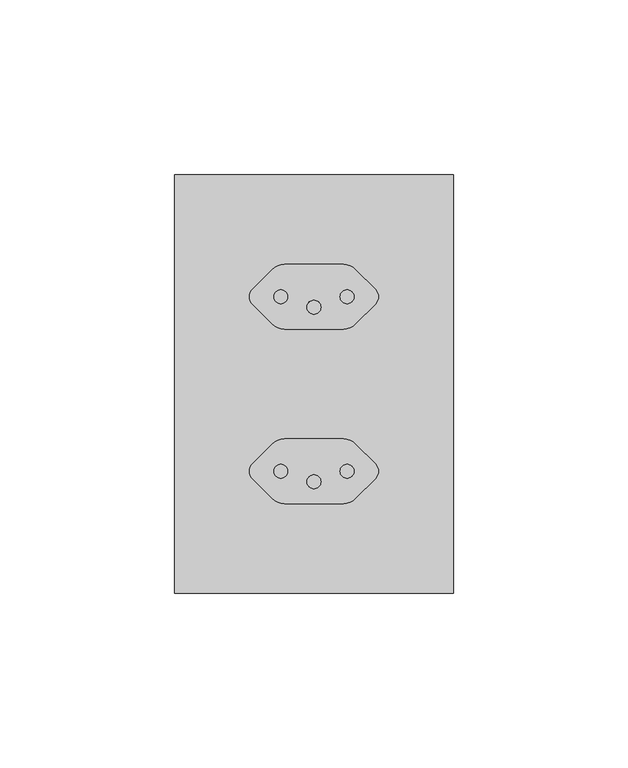
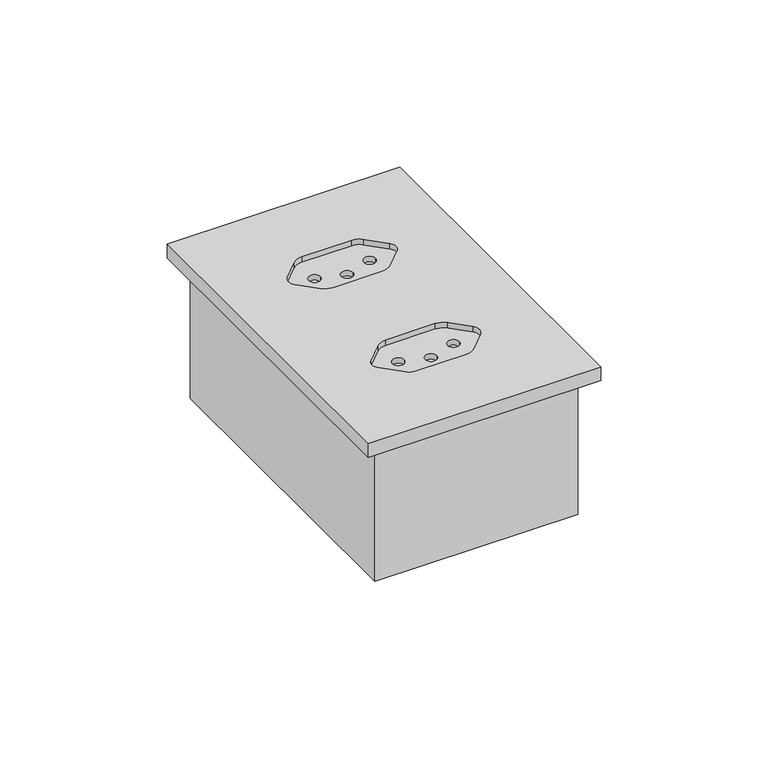
"""IFC4 building model written with IfcOpenShell, lengths in millimetres: proxy geometry, CAIXA VERTICE V7 : Tomada 10A 2s."""

import ifcopenshell
import ifcopenshell.guid

model = None  # the IFC model being written
_history = None  # IfcOwnerHistory: only IFC2X3 demands one
_inside = {}  # id of a spatial element -> (the spatial element, [elements in it])
_under = {}  # id of a project, library or spatial element -> (it, [spatial elements below it])
_declared = {}  # id of a project -> (the project, [libraries it declares])
_typed = {}  # id of a type object -> (the type object, [elements of that type])
_made_of = {}  # id of a material, layer set ... -> (it, [elements and type objects made of it])


def new_model(schema):
    """Start an empty IFC model of exactly this schema.

    Asked for "IFC4X3", IfcOpenShell would pick the latest addendum, in which some entities
    have other attributes; the version numbers below select the first issue.
    IFC2X3 requires an IfcOwnerHistory on every rooted entity: one is made here for all.
    """
    global model, _history
    if schema == "IFC4X3":
        model = ifcopenshell.file(schema_version=(4, 3, 0, 0))
    else:
        model = ifcopenshell.file(schema=schema)
    _inside.clear()
    _under.clear()
    _declared.clear()
    _typed.clear()
    _made_of.clear()
    _history = None
    if model.schema == "IFC2X3":
        org = make("IfcOrganization", Name="unknown")
        user = make(
            "IfcPersonAndOrganization",
            ThePerson=make("IfcPerson", FamilyName="unknown"),
            TheOrganization=org,
        )
        app = make(
            "IfcApplication",
            ApplicationDeveloper=org,
            Version="unknown",
            ApplicationFullName="unknown",
            ApplicationIdentifier="unknown",
        )
        _history = make(
            "IfcOwnerHistory",
            OwningUser=user,
            OwningApplication=app,
            ChangeAction="ADDED",
            CreationDate=0,
        )
    return model


def make(cls, **values):
    """One entity of the class cls with the attributes given. An attribute that is None is left unset."""
    return model.create_entity(
        cls, **{name: value for name, value in values.items() if value is not None}
    )


def rooted(cls, **values):
    """An entity with a GlobalId (a new one), such as an element, a storey or a relation."""
    return make(cls, GlobalId=ifcopenshell.guid.new(), OwnerHistory=_history, **values)


def si_unit(unit_type, name, prefix=None):
    """IfcSIUnit, for example si_unit("LENGTHUNIT", "METRE", prefix="MILLI")."""
    return make("IfcSIUnit", UnitType=unit_type, Prefix=prefix, Name=name)


def assignment(units):
    """IfcUnitAssignment: the units of a project."""
    return None if units is None else make("IfcUnitAssignment", Units=units)


def point(xyz):
    """IfcCartesianPoint."""
    return None if xyz is None else make("IfcCartesianPoint", Coordinates=xyz)


def direction(xyz):
    """IfcDirection."""
    return None if xyz is None else make("IfcDirection", DirectionRatios=xyz)


def frame(location, z_axis=None, x_axis=None):
    """IfcAxis2Placement3D, a coordinate frame: its origin and axes. An axis left out is left unset."""
    return make(
        "IfcAxis2Placement3D",
        Location=point(location),
        Axis=direction(z_axis),
        RefDirection=direction(x_axis),
    )


def origin():
    """The frame at (0, 0, 0) with its axes left unset."""
    return frame((0.0, 0.0, 0.0))


def place(relative_to, where):
    """IfcLocalPlacement: puts the frame where relative to a parent placement (None: the world)."""
    return make(
        "IfcLocalPlacement", PlacementRelTo=relative_to, RelativePlacement=where
    )


def context(
    kind, dimensions, precision=None, world=None, true_north=None, identifier=None
):
    """IfcGeometricRepresentationContext, for example the 3D "Model" context."""
    return make(
        "IfcGeometricRepresentationContext",
        ContextIdentifier=identifier,
        ContextType=kind,
        CoordinateSpaceDimension=dimensions,
        Precision=precision,
        WorldCoordinateSystem=world,
        TrueNorth=true_north,
    )


def project(units=None, contexts=None):
    """IfcProject with its units and contexts."""
    return rooted(
        "IfcProject",
        Name="project",
        RepresentationContexts=contexts,
        UnitsInContext=assignment(units),
    )


def spatial(cls, under=None, at=None, **own):
    """A site, building, storey or space (cls), placed at a placement, below another one or the project."""
    s = rooted(cls, ObjectPlacement=at, **own)
    if under is not None:
        _under.setdefault(under.id(), (under, []))[1].append(s)
    return s


def polyline(points):
    """IfcPolyline through the points."""
    return make("IfcPolyline", Points=[point(p) for p in points])


def circle_curve(where, radius):
    """IfcCircle in the frame where."""
    return make("IfcCircle", Position=where, Radius=radius)


def faces_of(points, faces, orient=None, outer=None):
    """IfcFace entities. A face is a list of loops; a loop is a list of indices into points, from 0.

    orient and outer hold one flag for each loop. By default every Orientation is true, the
    first loop of a face is its IfcFaceOuterBound and the others are IfcFaceBound.
    """
    made = []
    for i, loops in enumerate(faces):
        bounds = []
        for j, loop in enumerate(loops):
            is_outer = j == 0 if outer is None else outer[i][j]
            bounds.append(
                make(
                    "IfcFaceOuterBound" if is_outer else "IfcFaceBound",
                    Bound=make("IfcPolyLoop", Polygon=[points[k] for k in loop]),
                    Orientation=True if orient is None else orient[i][j],
                )
            )
        made.append(make("IfcFace", Bounds=bounds))
    return made


def faceted_brep(points, faces, orient=None, outer=None, voids=None):
    """IfcFacetedBrep: a solid bounded by flat faces; with voids (closed shells), ...WithVoids."""
    shared = [point(p) for p in points]
    hull = make("IfcClosedShell", CfsFaces=faces_of(shared, faces, orient, outer))
    if voids is None:
        return make("IfcFacetedBrep", Outer=hull)
    return make(
        "IfcFacetedBrepWithVoids",
        Outer=hull,
        Voids=[
            make(cls, CfsFaces=faces_of(shared, fs, o, b)) for cls, fs, o, b in voids
        ],
    )


def shape(context_of_items, identifier, shape_type, items):
    """IfcShapeRepresentation: the items that make up one representation, for example the "Body"."""
    return make(
        "IfcShapeRepresentation",
        ContextOfItems=context_of_items,
        RepresentationIdentifier=identifier,
        RepresentationType=shape_type,
        Items=items,
    )


def source(mapping_origin, context_of_items, identifier, shape_type, items):
    """IfcRepresentationMap: a shape defined once, which mapped items show again and again."""
    return make(
        "IfcRepresentationMap",
        MappingOrigin=mapping_origin,
        MappedRepresentation=shape(context_of_items, identifier, shape_type, items),
    )


def transform(
    local_origin,
    x_axis=None,
    y_axis=None,
    z_axis=None,
    scale=None,
    scale2=None,
    scale3=None,
    uniform=True,
):
    """IfcCartesianTransformationOperator3D, or its non-uniform kind. x_axis, y_axis, z_axis: its Axis1, 2, 3."""
    if uniform:
        return make(
            "IfcCartesianTransformationOperator3D",
            Axis1=direction(x_axis),
            Axis2=direction(y_axis),
            LocalOrigin=point(local_origin),
            Scale=scale,
            Axis3=direction(z_axis),
        )
    return make(
        "IfcCartesianTransformationOperator3DnonUniform",
        Axis1=direction(x_axis),
        Axis2=direction(y_axis),
        LocalOrigin=point(local_origin),
        Scale=scale,
        Axis3=direction(z_axis),
        Scale2=scale2,
        Scale3=scale3,
    )


def mapped(mapping_source, mapping_target):
    """IfcMappedItem: shows the shape of a source again, moved by a transform."""
    return make(
        "IfcMappedItem", MappingSource=mapping_source, MappingTarget=mapping_target
    )


def made_of(thing, what):
    """Note that an element or type object is made of a material, layer set ...; save() writes the relation."""
    if what is not None:
        _made_of.setdefault(what.id(), (what, []))[1].append(thing)
    return thing


def element(
    cls,
    number,
    at=None,
    inside=None,
    cuts=None,
    type_object=None,
    material=None,
    context=None,
    identifier="Body",
    shape_type=None,
    held_by="IfcProductDefinitionShape",
    body=None,
    shapes=None,
    **own,
):
    """One element of the class cls, such as IfcWall. Its Tag is "e" and its number.

    at: its placement. inside: the storey or other place that contains it. cuts: it is an
    opening in that element (IfcRelVoidsElement). A single representation is given by context,
    identifier, shape_type and body (its items); several are given by shapes. held_by: the class
    of the entity that holds the representations. save() writes the other relations.
    """
    e = rooted(cls, Tag="e%d" % number, ObjectPlacement=at, **own)
    if body is not None:
        shapes = [shape(context, identifier, shape_type, body)]
    if shapes is not None:
        e.Representation = make(held_by, Representations=shapes)
    if inside is not None:
        _inside.setdefault(inside.id(), (inside, []))[1].append(e)
    if cuts is not None:
        rooted(
            "IfcRelVoidsElement", RelatingBuildingElement=cuts, RelatedOpeningElement=e
        )
    if type_object is not None:
        _typed.setdefault(type_object.id(), (type_object, []))[1].append(e)
    return made_of(e, material)


def aggregate(whole, parts):
    """IfcRelAggregates: a whole, such as a stair, and the parts it consists of."""
    return rooted("IfcRelAggregates", RelatingObject=whole, RelatedObjects=parts)


def save(model, path):
    """Write the relations noted so far, then the file.

    IfcRelAggregates (storeys below a building ...), IfcRelContainedInSpatialStructure (elements
    in a storey), IfcRelDefinesByType, IfcRelAssociatesMaterial and IfcRelDeclares: one each for
    every whole, place, type object, material and project.
    """
    for whole, parts in _under.values():
        aggregate(whole, parts)
    for where, things in _inside.values():
        rooted(
            "IfcRelContainedInSpatialStructure",
            RelatedElements=things,
            RelatingStructure=where,
        )
    for kind, things in _typed.values():
        rooted("IfcRelDefinesByType", RelatedObjects=things, RelatingType=kind)
    for what, things in _made_of.values():
        rooted("IfcRelAssociatesMaterial", RelatedObjects=things, RelatingMaterial=what)
    for by, libraries in _declared.values():
        rooted("IfcRelDeclares", RelatingContext=by, RelatedDefinitions=libraries)
    model.write(path)


def plane_surface(at):
    """IfcPlane: the flat surface through the origin of the frame at, square to its z axis."""
    return make("IfcPlane", Position=at)


def revolved_surface(curve, axis_point, axis_direction):
    """IfcSurfaceOfRevolution: the curve turned about the line through axis_point along axis_direction."""
    return make(
        "IfcSurfaceOfRevolution",
        SweptCurve=make("IfcArbitraryOpenProfileDef", ProfileType="CURVE", Curve=curve),
        AxisPosition=make("IfcAxis1Placement", Location=point(axis_point), Axis=direction(axis_direction)),
    )


def advanced_brep(points, edges, surfaces, faces):
    """IfcAdvancedBrep: a solid bounded by faces that lie on surfaces and meet in shared edges.

    An edge is (start, end): straight between two places in points (the first is 0);
    or (start, end, curve); or (start, end, curve, False) where it runs against its curve.
    A face is (place in surfaces, loops), or (place, loops, False) where it looks against
    its surface's normal. A loop lists edges by number (the first is 1), with a minus sign
    where the edge is run from its end to its start. The first loop is the outer one.
    """
    corners = [point(p) for p in points]
    vertices = [make("IfcVertexPoint", VertexGeometry=c) for c in corners]
    made = []
    for start, end, *more in edges:
        made.append(
            make(
                "IfcEdgeCurve",
                EdgeStart=vertices[start],
                EdgeEnd=vertices[end],
                EdgeGeometry=more[0] if more else make("IfcPolyline", Points=[corners[start], corners[end]]),
                SameSense=more[1] if len(more) > 1 else True,
            )
        )
    hull = []
    for where, loops, *sense in faces:
        bounds = []
        for j, loop in enumerate(loops):
            ring = [make("IfcOrientedEdge", EdgeElement=made[abs(k) - 1], Orientation=k > 0) for k in loop]
            bounds.append(
                make(
                    "IfcFaceOuterBound" if j == 0 else "IfcFaceBound",
                    Bound=make("IfcEdgeLoop", EdgeList=ring),
                    Orientation=True,
                )
            )
        hull.append(make("IfcAdvancedFace", Bounds=bounds, FaceSurface=surfaces[where], SameSense=sense[0] if sense else True))
    return make("IfcAdvancedBrep", Outer=make("IfcClosedShell", CfsFaces=hull))


def electrical_fixtures_8aeb2822(model_context):
    return source(origin(), model_context, "Body", "SolidModel", [
        faceted_brep([(33.0, -247.0, -48.0), (-33.0, -247.0, -48.0), (-33.0, -353.0, -48.0), (33.0, -353.0, -48.0), (35.0, -355.0, -50.0), (-35.0, -355.0, -50.0), (-35.0, -245.0, -50.0), (35.0, -245.0, -50.0), (35.0, -355.0, 0.0), (-35.0, -355.0, 0.0), (-35.0, -245.0, 0.0), (35.0, -245.0, 0.0), (33.0, -353.0, 0.0), (-33.0, -353.0, 0.0), (-33.0, -247.0, 0.0), (33.0, -247.0, 0.0)], [[[0, 1, 2, 3]], [[4, 5, 6, 7]], [[4, 8, 9, 5]], [[9, 10, 6, 5]], [[10, 11, 7, 6]], [[11, 8, 4, 7]], [[8, 11, 10, 9], [12, 13, 14, 15]], [[15, 0, 3, 12]], [[14, 1, 0, 15]], [[13, 2, 1, 14]], [[12, 3, 2, 13]]]),
        advanced_brep(
        [(40.0, -360.0, 5.0), (40.0, -240.0, 5.0), (-40.0, -240.0, 5.0), (-40.0, -360.0, 5.0), (8.4215729, -315.75, 5.0), (11.9571068, -317.2144661, 5.0), (17.6213203, -322.8786797, 5.0), (17.6213203, -327.1213203, 5.0), (11.9571068, -332.7855339, 5.0), (8.4215729, -334.25, 5.0), (-8.4215729, -334.25, 5.0), (-11.9571068, -332.7855339, 5.0), (-17.6213203, -327.1213203, 5.0), (-17.6213203, -322.8786797, 5.0), (-11.9571068, -317.2144661, 5.0), (-8.4215729, -315.75, 5.0), (8.4215729, -265.75, 5.0), (11.9571068, -267.2144661, 5.0), (17.6213203, -272.8786797, 5.0), (17.6213203, -277.1213203, 5.0), (11.9571068, -282.7855339, 5.0), (8.4215729, -284.25, 5.0), (-8.4215729, -284.25, 5.0), (-11.9571068, -282.7855339, 5.0), (-17.6213203, -277.1213203, 5.0), (-17.6213203, -272.8786797, 5.0), (-11.9571068, -267.2144661, 5.0), (-8.4215729, -265.75, 5.0), (-40.0, -360.0, 0.0), (-40.0, -240.0, 0.0), (40.0, -240.0, 0.0), (40.0, -360.0, 0.0), (8.4215729, -315.75, 3.0), (-8.4215729, -315.75, 3.0), (-11.9571068, -317.2144661, 3.0), (-17.6213203, -322.8786797, 3.0), (-17.6213203, -327.1213203, 3.0), (-11.9571068, -332.7855339, 3.0), (-8.4215729, -334.25, 3.0), (8.4215729, -334.25, 3.0), (11.9571068, -332.7855339, 3.0), (17.6213203, -327.1213203, 3.0), (17.6213203, -322.8786797, 3.0), (11.9571068, -317.2144661, 3.0), (-7.5, -325.0, 3.0), (-11.5, -325.0, 3.0), (11.5, -325.0, 3.0), (7.5, -325.0, 3.0), (2.0, -328.0, 3.0), (-2.0, -328.0, 3.0), (-11.5, -325.0, 1.0), (-7.5, -325.0, 1.0), (7.5, -325.0, 1.0), (11.5, -325.0, 1.0), (-2.0, -328.0, 1.0), (2.0, -328.0, 1.0), (8.4215729, -265.75, 3.0), (-8.4215729, -265.75, 3.0), (-11.9571068, -267.2144661, 3.0), (-17.6213203, -272.8786797, 3.0), (-17.6213203, -277.1213203, 3.0), (-11.9571068, -282.7855339, 3.0), (-8.4215729, -284.25, 3.0), (8.4215729, -284.25, 3.0), (11.9571068, -282.7855339, 3.0), (17.6213203, -277.1213203, 3.0), (17.6213203, -272.8786797, 3.0), (11.9571068, -267.2144661, 3.0), (-7.5, -275.0, 3.0), (-11.5, -275.0, 3.0), (11.5, -275.0, 3.0), (7.5, -275.0, 3.0), (2.0, -278.0, 3.0), (-2.0, -278.0, 3.0), (-11.5, -275.0, 1.0), (-7.5, -275.0, 1.0), (7.5, -275.0, 1.0), (11.5, -275.0, 1.0), (-2.0, -278.0, 1.0), (2.0, -278.0, 1.0)],
        [
            (0, 1),
            (1, 2),
            (2, 3),
            (3, 0),
            (4, 5, circle_curve(frame((8.4215729, -320.75, 5.0), z_axis=(0.0, 0.0, -1.0), x_axis=(-1.0, 0.0, 0.0)), 5.0)),
            (5, 6),
            (6, 7, circle_curve(frame((15.5, -325.0, 5.0), z_axis=(0.0, 0.0, -1.0), x_axis=(-1.0, 0.0, 0.0)), 3.0)),
            (7, 8),
            (8, 9, circle_curve(frame((8.4215729, -329.25, 5.0), z_axis=(0.0, 0.0, -1.0), x_axis=(-1.0, 0.0, 0.0)), 5.0)),
            (9, 10),
            (10, 11, circle_curve(frame((-8.4215729, -329.25, 5.0), z_axis=(0.0, 0.0, -1.0), x_axis=(-1.0, 0.0, 0.0)), 5.0)),
            (11, 12),
            (12, 13, circle_curve(frame((-15.5, -325.0, 5.0), z_axis=(0.0, 0.0, -1.0), x_axis=(-1.0, 0.0, 0.0)), 3.0)),
            (13, 14),
            (14, 15, circle_curve(frame((-8.4215729, -320.75, 5.0), z_axis=(0.0, 0.0, -1.0), x_axis=(-1.0, 0.0, 0.0)), 5.0)),
            (15, 4),
            (16, 17, circle_curve(frame((8.4215729, -270.75, 5.0), z_axis=(0.0, 0.0, -1.0), x_axis=(-1.0, 0.0, 0.0)), 5.0)),
            (17, 18),
            (18, 19, circle_curve(frame((15.5, -275.0, 5.0), z_axis=(0.0, 0.0, -1.0), x_axis=(-1.0, 0.0, 0.0)), 3.0)),
            (19, 20),
            (20, 21, circle_curve(frame((8.4215729, -279.25, 5.0), z_axis=(0.0, 0.0, -1.0), x_axis=(-1.0, 0.0, 0.0)), 5.0)),
            (21, 22),
            (22, 23, circle_curve(frame((-8.4215729, -279.25, 5.0), z_axis=(0.0, 0.0, -1.0), x_axis=(-1.0, 0.0, 0.0)), 5.0)),
            (23, 24),
            (24, 25, circle_curve(frame((-15.5, -275.0, 5.0), z_axis=(0.0, 0.0, -1.0), x_axis=(-1.0, 0.0, 0.0)), 3.0)),
            (25, 26),
            (26, 27, circle_curve(frame((-8.4215729, -270.75, 5.0), z_axis=(0.0, 0.0, -1.0), x_axis=(-1.0, 0.0, 0.0)), 5.0)),
            (27, 16),
            (28, 29),
            (29, 30),
            (30, 31),
            (31, 28),
            (3, 28),
            (31, 0),
            (2, 29),
            (1, 30),
            (32, 33),
            (33, 34, circle_curve(frame((-8.4215729, -320.75, 3.0), z_axis=(0.0, 0.0, 1.0), x_axis=(-1.0, 0.0, 0.0)), 5.0)),
            (34, 35),
            (35, 36, circle_curve(frame((-15.5, -325.0, 3.0), z_axis=(0.0, 0.0, 1.0), x_axis=(-1.0, 0.0, 0.0)), 3.0)),
            (36, 37),
            (37, 38, circle_curve(frame((-8.4215729, -329.25, 3.0), z_axis=(0.0, 0.0, 1.0), x_axis=(-1.0, 0.0, 0.0)), 5.0)),
            (38, 39),
            (39, 40, circle_curve(frame((8.4215729, -329.25, 3.0), z_axis=(0.0, 0.0, 1.0), x_axis=(-1.0, 0.0, 0.0)), 5.0)),
            (40, 41),
            (41, 42, circle_curve(frame((15.5, -325.0, 3.0), z_axis=(0.0, 0.0, 1.0), x_axis=(-1.0, 0.0, 0.0)), 3.0)),
            (42, 43),
            (43, 32, circle_curve(frame((8.4215729, -320.75, 3.0), z_axis=(0.0, 0.0, 1.0), x_axis=(-1.0, 0.0, 0.0)), 5.0)),
            (44, 45, circle_curve(frame((-9.5, -325.0, 3.0), z_axis=(0.0, 0.0, -1.0), x_axis=(1.0, -2.301812013077709e-12, 0.0)), 2.0)),
            (45, 44, circle_curve(frame((-9.5, -325.0, 3.0), z_axis=(0.0, 0.0, -1.0), x_axis=(1.0, -2.301812013077709e-12, 0.0)), 2.0)),
            (46, 47, circle_curve(frame((9.5, -325.0, 3.0), z_axis=(0.0, 0.0, -1.0), x_axis=(1.0, -2.301812013077709e-12, 0.0)), 2.0)),
            (47, 46, circle_curve(frame((9.5, -325.0, 3.0), z_axis=(0.0, 0.0, -1.0), x_axis=(1.0, -2.301812013077709e-12, 0.0)), 2.0)),
            (48, 49, circle_curve(frame((0.0, -328.0, 3.0), z_axis=(0.0, 0.0, -1.0), x_axis=(1.0, -2.301812013077709e-12, 0.0)), 2.0)),
            (49, 48, circle_curve(frame((0.0, -328.0, 3.0), z_axis=(0.0, 0.0, -1.0), x_axis=(1.0, -2.301812013077709e-12, 0.0)), 2.0)),
            (32, 4),
            (15, 33),
            (14, 34),
            (13, 35),
            (12, 36),
            (11, 37),
            (10, 38),
            (9, 39),
            (8, 40),
            (7, 41),
            (6, 42),
            (5, 43),
            (50, 51, circle_curve(frame((-9.5, -325.0, 1.0), z_axis=(0.0, 0.0, 1.0), x_axis=(1.0, -2.301812013077709e-12, 0.0)), 2.0)),
            (51, 50, circle_curve(frame((-9.5, -325.0, 1.0), z_axis=(0.0, 0.0, 1.0), x_axis=(1.0, -2.301812013077709e-12, 0.0)), 2.0)),
            (52, 53, circle_curve(frame((9.5, -325.0, 1.0), z_axis=(0.0, 0.0, 1.0), x_axis=(1.0, -2.301812013077709e-12, 0.0)), 2.0)),
            (53, 52, circle_curve(frame((9.5, -325.0, 1.0), z_axis=(0.0, 0.0, 1.0), x_axis=(1.0, -2.301812013077709e-12, 0.0)), 2.0)),
            (54, 55, circle_curve(frame((0.0, -328.0, 1.0), z_axis=(0.0, 0.0, 1.0), x_axis=(1.0, -2.301812013077709e-12, 0.0)), 2.0)),
            (55, 54, circle_curve(frame((0.0, -328.0, 1.0), z_axis=(0.0, 0.0, 1.0), x_axis=(1.0, -2.301812013077709e-12, 0.0)), 2.0)),
            (45, 50),
            (51, 44),
            (47, 52),
            (53, 46),
            (49, 54),
            (55, 48),
            (56, 57),
            (57, 58, circle_curve(frame((-8.4215729, -270.75, 3.0), z_axis=(0.0, 0.0, 1.0), x_axis=(-1.0, 0.0, 0.0)), 5.0)),
            (58, 59),
            (59, 60, circle_curve(frame((-15.5, -275.0, 3.0), z_axis=(0.0, 0.0, 1.0), x_axis=(-1.0, 0.0, 0.0)), 3.0)),
            (60, 61),
            (61, 62, circle_curve(frame((-8.4215729, -279.25, 3.0), z_axis=(0.0, 0.0, 1.0), x_axis=(-1.0, 0.0, 0.0)), 5.0)),
            (62, 63),
            (63, 64, circle_curve(frame((8.4215729, -279.25, 3.0), z_axis=(0.0, 0.0, 1.0), x_axis=(-1.0, 0.0, 0.0)), 5.0)),
            (64, 65),
            (65, 66, circle_curve(frame((15.5, -275.0, 3.0), z_axis=(0.0, 0.0, 1.0), x_axis=(-1.0, 0.0, 0.0)), 3.0)),
            (66, 67),
            (67, 56, circle_curve(frame((8.4215729, -270.75, 3.0), z_axis=(0.0, 0.0, 1.0), x_axis=(-1.0, 0.0, 0.0)), 5.0)),
            (68, 69, circle_curve(frame((-9.5, -275.0, 3.0), z_axis=(0.0, 0.0, -1.0), x_axis=(1.0, -2.301812013077709e-12, 0.0)), 2.0)),
            (69, 68, circle_curve(frame((-9.5, -275.0, 3.0), z_axis=(0.0, 0.0, -1.0), x_axis=(1.0, -2.301812013077709e-12, 0.0)), 2.0)),
            (70, 71, circle_curve(frame((9.5, -275.0, 3.0), z_axis=(0.0, 0.0, -1.0), x_axis=(1.0, -2.301812013077709e-12, 0.0)), 2.0)),
            (71, 70, circle_curve(frame((9.5, -275.0, 3.0), z_axis=(0.0, 0.0, -1.0), x_axis=(1.0, -2.301812013077709e-12, 0.0)), 2.0)),
            (72, 73, circle_curve(frame((0.0, -278.0, 3.0), z_axis=(0.0, 0.0, -1.0), x_axis=(1.0, -2.301812013077709e-12, 0.0)), 2.0)),
            (73, 72, circle_curve(frame((0.0, -278.0, 3.0), z_axis=(0.0, 0.0, -1.0), x_axis=(1.0, -2.301812013077709e-12, 0.0)), 2.0)),
            (56, 16),
            (27, 57),
            (26, 58),
            (25, 59),
            (24, 60),
            (23, 61),
            (22, 62),
            (21, 63),
            (20, 64),
            (19, 65),
            (18, 66),
            (17, 67),
            (74, 75, circle_curve(frame((-9.5, -275.0, 1.0), z_axis=(0.0, 0.0, 1.0), x_axis=(1.0, -2.301812013077709e-12, 0.0)), 2.0)),
            (75, 74, circle_curve(frame((-9.5, -275.0, 1.0), z_axis=(0.0, 0.0, 1.0), x_axis=(1.0, -2.301812013077709e-12, 0.0)), 2.0)),
            (76, 77, circle_curve(frame((9.5, -275.0, 1.0), z_axis=(0.0, 0.0, 1.0), x_axis=(1.0, -2.301812013077709e-12, 0.0)), 2.0)),
            (77, 76, circle_curve(frame((9.5, -275.0, 1.0), z_axis=(0.0, 0.0, 1.0), x_axis=(1.0, -2.301812013077709e-12, 0.0)), 2.0)),
            (78, 79, circle_curve(frame((0.0, -278.0, 1.0), z_axis=(0.0, 0.0, 1.0), x_axis=(1.0, -2.301812013077709e-12, 0.0)), 2.0)),
            (79, 78, circle_curve(frame((0.0, -278.0, 1.0), z_axis=(0.0, 0.0, 1.0), x_axis=(1.0, -2.301812013077709e-12, 0.0)), 2.0)),
            (69, 74),
            (75, 68),
            (71, 76),
            (77, 70),
            (73, 78),
            (79, 72),
        ],
        [
            plane_surface(frame((-60.0, -360.0, 5.0), z_axis=(0.0, 0.0, 1.0), x_axis=(-1.0, 0.0, 0.0))),
            plane_surface(frame((-60.0, -360.0, 0.0), z_axis=(0.0, 0.0, -1.0), x_axis=(1.0, 0.0, 0.0))),
            plane_surface(frame((40.0, -360.0, 5.0), z_axis=(0.0, -1.0, 0.0), x_axis=(0.0, 0.0, -1.0))),
            plane_surface(frame((-40.0, -360.0, 5.0), z_axis=(-1.0, 0.0, 0.0), x_axis=(0.0, 0.0, -1.0))),
            plane_surface(frame((-40.0, -240.0, 5.0), z_axis=(0.0, 1.0, 0.0), x_axis=(0.0, 0.0, -1.0))),
            plane_surface(frame((40.0, -240.0, 5.0), z_axis=(1.0, 0.0, 0.0), x_axis=(0.0, 0.0, -1.0))),
            plane_surface(frame((3.4215729, -320.75, 3.0), z_axis=(0.0, 0.0, 1.0), x_axis=(0.0, -1.0, 0.0))),
            plane_surface(frame((-8.4215729, -315.75, 5.0), z_axis=(0.0, -1.0, 0.0), x_axis=(0.0, 0.0, -1.0))),
            revolved_surface(polyline([(-13.4215729, -320.75, 5.0), (-13.4215729, -320.75, 3.0)]), (-8.4215729, -320.75, 3.0), (0.0, 0.0, 1.0)),
            plane_surface(frame((-17.6213203, -322.8786797, 5.0), z_axis=(0.7071067811865045, -0.7071067811865905, 0.0), x_axis=(0.0, 0.0, -1.0))),
            revolved_surface(polyline([(-18.5, -325.0, 5.0), (-18.5, -325.0, 3.0)]), (-15.5, -325.0, 3.0), (0.0, 0.0, 1.0)),
            plane_surface(frame((-11.9571068, -332.7855339, 5.0), z_axis=(0.7071067811865515, 0.7071067811865437, 0.0), x_axis=(0.0, 0.0, -1.0))),
            revolved_surface(polyline([(-13.4215729, -329.25, 5.0), (-13.4215729, -329.25, 3.0)]), (-8.4215729, -329.25, 3.0), (0.0, 0.0, 1.0)),
            plane_surface(frame((8.4215729, -334.25, 5.0), z_axis=(0.0, 1.0, 0.0), x_axis=(0.0, 0.0, -1.0))),
            revolved_surface(polyline([(3.4215728999999993, -329.25, 5.0), (3.4215728999999993, -329.25, 3.0)]), (8.4215729, -329.25, 3.0), (0.0, 0.0, 1.0)),
            plane_surface(frame((17.6213203, -327.1213203, 5.0), z_axis=(-0.7071067811865307, 0.7071067811865643, 0.0), x_axis=(0.0, 0.0, -1.0))),
            revolved_surface(polyline([(12.5, -325.0, 5.0), (12.5, -325.0, 3.0)]), (15.5, -325.0, 3.0), (0.0, 0.0, 1.0)),
            plane_surface(frame((11.9571068, -317.2144661, 5.0), z_axis=(-0.7071067811865893, -0.7071067811865058, 0.0), x_axis=(0.0, 0.0, -1.0))),
            revolved_surface(polyline([(3.4215728999999993, -320.75, 5.0), (3.4215728999999993, -320.75, 3.0)]), (8.4215729, -320.75, 3.0), (0.0, 0.0, 1.0)),
            plane_surface(frame((-7.5, -325.0, 1.0), z_axis=(0.0, 0.0, 1.0), x_axis=(2.301812013077709e-12, 1.0, 0.0))),
            revolved_surface(polyline([(-7.5, -325.0000000000046, 3.0), (-7.5, -325.0000000000046, 1.0)]), (-9.5, -325.0, 1.0), (0.0, 0.0, 1.0)),
            revolved_surface(polyline([(11.5, -325.0000000000046, 3.0), (11.5, -325.0000000000046, 1.0)]), (9.5, -325.0, 5.0), (0.0, 0.0, 1.0)),
            revolved_surface(polyline([(2.0, -328.0000000000046, 3.0), (2.0, -328.0000000000046, 1.0)]), (0.0, -328.0, 5.0), (0.0, 0.0, 1.0)),
            plane_surface(frame((3.4215729, -270.75, 3.0), z_axis=(0.0, 0.0, 1.0), x_axis=(0.0, -1.0, 0.0))),
            plane_surface(frame((-8.4215729, -265.75, 5.0), z_axis=(0.0, -1.0, 0.0), x_axis=(0.0, 0.0, -1.0))),
            revolved_surface(polyline([(-13.4215729, -270.75, 5.0), (-13.4215729, -270.75, 3.0)]), (-8.4215729, -270.75, 3.0), (0.0, 0.0, 1.0)),
            plane_surface(frame((-17.6213203, -272.8786797, 5.0), z_axis=(0.7071067811865045, -0.7071067811865905, 0.0), x_axis=(0.0, 0.0, -1.0))),
            revolved_surface(polyline([(-18.5, -275.0, 5.0), (-18.5, -275.0, 3.0)]), (-15.5, -275.0, 3.0), (0.0, 0.0, 1.0)),
            plane_surface(frame((-11.9571068, -282.7855339, 5.0), z_axis=(0.7071067811865515, 0.7071067811865437, 0.0), x_axis=(0.0, 0.0, -1.0))),
            revolved_surface(polyline([(-13.4215729, -279.25, 5.0), (-13.4215729, -279.25, 3.0)]), (-8.4215729, -279.25, 3.0), (0.0, 0.0, 1.0)),
            plane_surface(frame((8.4215729, -284.25, 5.0), z_axis=(0.0, 1.0, 0.0), x_axis=(0.0, 0.0, -1.0))),
            revolved_surface(polyline([(3.4215728999999993, -279.25, 5.0), (3.4215728999999993, -279.25, 3.0)]), (8.4215729, -279.25, 3.0), (0.0, 0.0, 1.0)),
            plane_surface(frame((17.6213203, -277.1213203, 5.0), z_axis=(-0.7071067811865307, 0.7071067811865643, 0.0), x_axis=(0.0, 0.0, -1.0))),
            revolved_surface(polyline([(12.5, -275.0, 5.0), (12.5, -275.0, 3.0)]), (15.5, -275.0, 3.0), (0.0, 0.0, 1.0)),
            plane_surface(frame((11.9571068, -267.2144661, 5.0), z_axis=(-0.7071067811865893, -0.7071067811865058, 0.0), x_axis=(0.0, 0.0, -1.0))),
            revolved_surface(polyline([(3.4215728999999993, -270.75, 5.0), (3.4215728999999993, -270.75, 3.0)]), (8.4215729, -270.75, 3.0), (0.0, 0.0, 1.0)),
            plane_surface(frame((-7.5, -275.0, 1.0), z_axis=(0.0, 0.0, 1.0), x_axis=(2.301812013077709e-12, 1.0, 0.0))),
            revolved_surface(polyline([(-7.5, -275.0000000000046, 3.0), (-7.5, -275.0000000000046, 1.0)]), (-9.5, -275.0, 1.0), (0.0, 0.0, 1.0)),
            revolved_surface(polyline([(11.5, -275.0000000000046, 3.0), (11.5, -275.0000000000046, 1.0)]), (9.5, -275.0, 5.0), (0.0, 0.0, 1.0)),
            revolved_surface(polyline([(2.0, -278.0000000000046, 3.0), (2.0, -278.0000000000046, 1.0)]), (0.0, -278.0, 5.0), (0.0, 0.0, 1.0)),
        ],
        [
            (0, [[1, 2, 3, 4], [5, 6, 7, 8, 9, 10, 11, 12, 13, 14, 15, 16], [17, 18, 19, 20, 21, 22, 23, 24, 25, 26, 27, 28]]),
            (1, [[29, 30, 31, 32]]),
            (2, [[33, -32, 34, -4]]),
            (3, [[35, -29, -33, -3]]),
            (4, [[36, -30, -35, -2]]),
            (5, [[-34, -31, -36, -1]]),
            (6, [[37, 38, 39, 40, 41, 42, 43, 44, 45, 46, 47, 48], [49, 50], [51, 52], [53, 54]]),
            (7, [[55, -16, 56, -37]]),
            (8, [[-56, -15, 57, -38]]),
            (9, [[-57, -14, 58, -39]]),
            (10, [[-58, -13, 59, -40]]),
            (11, [[-59, -12, 60, -41]]),
            (12, [[-60, -11, 61, -42]]),
            (13, [[-61, -10, 62, -43]]),
            (14, [[-62, -9, 63, -44]]),
            (15, [[-63, -8, 64, -45]]),
            (16, [[-64, -7, 65, -46]]),
            (17, [[-65, -6, 66, -47]]),
            (18, [[-66, -5, -55, -48]]),
            (19, [[67, 68]]),
            (19, [[69, 70]]),
            (19, [[71, 72]]),
            (20, [[73, -68, 74, -50]]),
            (20, [[-74, -67, -73, -49]]),
            (21, [[75, -70, 76, -52]]),
            (21, [[-76, -69, -75, -51]]),
            (22, [[77, -72, 78, -54]]),
            (22, [[-78, -71, -77, -53]]),
            (23, [[79, 80, 81, 82, 83, 84, 85, 86, 87, 88, 89, 90], [91, 92], [93, 94], [95, 96]]),
            (24, [[97, -28, 98, -79]]),
            (25, [[-98, -27, 99, -80]]),
            (26, [[-99, -26, 100, -81]]),
            (27, [[-100, -25, 101, -82]]),
            (28, [[-101, -24, 102, -83]]),
            (29, [[-102, -23, 103, -84]]),
            (30, [[-103, -22, 104, -85]]),
            (31, [[-104, -21, 105, -86]]),
            (32, [[-105, -20, 106, -87]]),
            (33, [[-106, -19, 107, -88]]),
            (34, [[-107, -18, 108, -89]]),
            (35, [[-108, -17, -97, -90]]),
            (36, [[109, 110]]),
            (36, [[111, 112]]),
            (36, [[113, 114]]),
            (37, [[115, -110, 116, -92]]),
            (37, [[-116, -109, -115, -91]]),
            (38, [[117, -112, 118, -94]]),
            (38, [[-118, -111, -117, -93]]),
            (39, [[119, -114, 120, -96]]),
            (39, [[-120, -113, -119, -95]]),
        ],
    ),
    ])


if __name__ == "__main__":
    model = new_model("IFC4")
    model_context = context("Model", 3, world=origin())
    ifc_project = project(units=[si_unit("LENGTHUNIT", "METRE", prefix="MILLI")], contexts=[model_context])
    site = spatial("IfcSite", under=ifc_project)
    building = spatial("IfcBuilding", under=site)
    placement = place(None, origin())
    electrical_fixtures_shape = electrical_fixtures_8aeb2822(model_context)
    element("IfcBuildingElementProxy", 1, Name="CAIXA VERTICE V7 : Tomada 10A 2s", ObjectType="CAIXA VERTICE V7 : Tomada 10A 2s", at=placement, inside=building, context=model_context, shape_type="MappedRepresentation", body=[
        mapped(electrical_fixtures_shape, transform((0.0, 0.0, 0.0), x_axis=(1.0, 0.0, 0.0), y_axis=(0.0, 1.0, 0.0), z_axis=(0.0, 0.0, 1.0))),
    ])
    save(model, "model.ifc")

# Revit data of these elements
# Type "CAIXA VERTICE V7 : Tomada 10A 2s"
#   URL = "www.facebook.com/verticetreinamentos"
#   SEÇÃO [instance default] = ""
#   Rotação [instance default] = 0.00°
#   LARGURA DA TAMPA = 0.08 m
#   BORDA = 0.01 m
#   ALTURA DE INSTALAÇÃO [instance default] = 1.10 m
#   Distância Anotação [instance default] = 0.0015 m
#   ALTURA DA TAMPA = 0.12 m
#   Vertical [instance default] = yes
#   VER SEÇÃO [instance default] = no
#   SHADE ESQ [instance default] = no
#   SHADE DIR [instance default] = yes
#   HORIZONTAL [instance default] = no
#   ANDAR COM A LEGENDA [instance default] = 0
#   Material Tampa [instance default] = Plástico, branco opaco
#   Caixa = element 1798515
#   Anotação = element 1798529
#   Default Elevation = 0
# Element 1 (IfcBuildingElementProxy, "CAIXA VERTICE V7 : Tomada 10A 2s")
#   ALTURA DE INSTALAÇÃO = 0.30 m
#   SHADE DIR = no
#   Materials on its faces: "Plástico, branco opaco"
# Materials
#   "Plástico, branco opaco": class "Plástico", colour RGB 120 120 120, transparency 0, Description = "Plastic, generic, opaque white", Cost = 0
